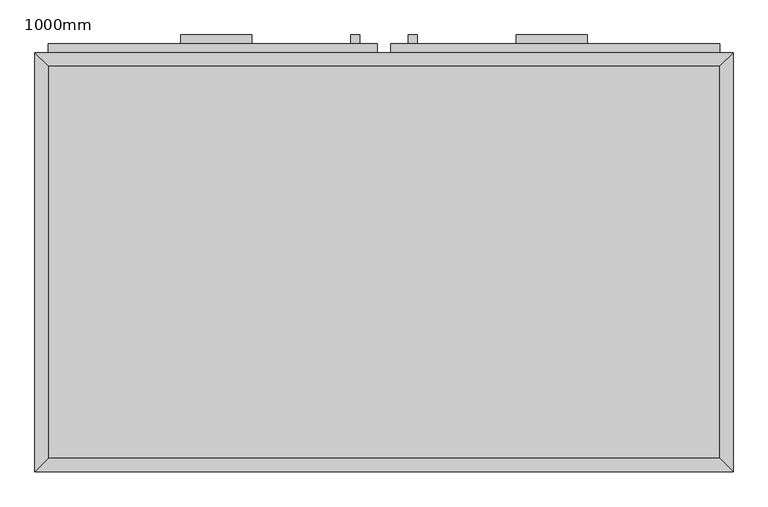
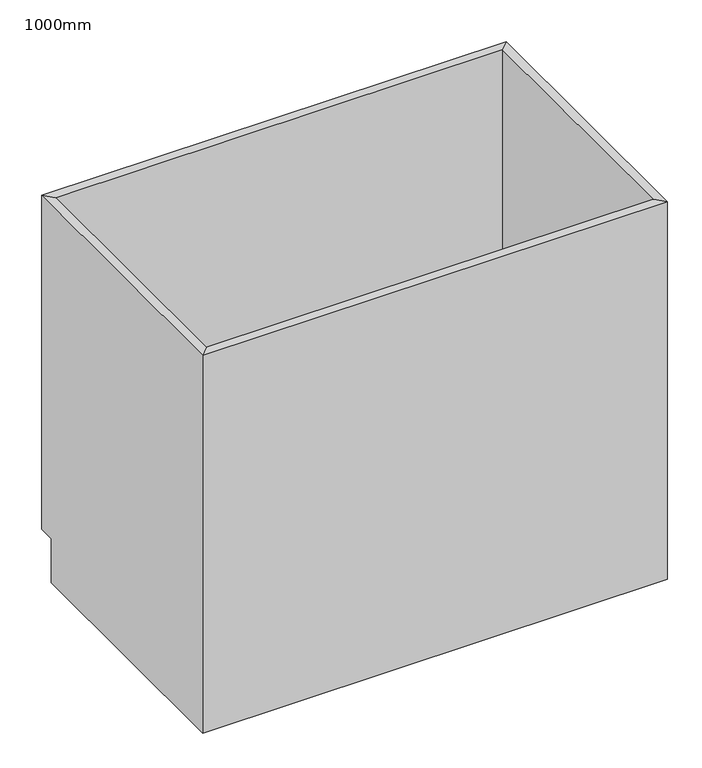
"""IFC4 building model written with IfcOpenShell, lengths in millimetres: furniture geometry, M_Base Cabinet-Double Door & 2 Drawer : 1000mm."""

from ifc_helpers import new_model, si_unit, frame, origin, place, context, project, spatial, polyline, outline, extrude, faceted_brep, source, transform, mapped, element, save


def furniture_1000mm_55825455(model_context):
    return source(origin(), model_context, "Body", "SolidModel", [
        faceted_brep([(499.6877049, 580.95, 860.0), (-462.2122951, 580.95, 860.0), (-462.2122951, 580.95, 100.0), (499.6877049, 580.95, 100.0), (518.7377049, 600.0, 860.0), (-481.2622951, 600.0, 860.0), (518.7377049, 600.0, 100.0), (-481.2622951, 600.0, 100.0), (-462.2122951, 19.05, 860.0), (-462.2122951, 19.05, 100.0), (-462.2122951, 565.0, 100.0), (-481.2622951, 0.0, 860.0), (-481.2622951, 565.0, 100.0), (-481.2622951, 565.0, 0.0), (-481.2622951, 0.0, 0.0), (499.6877049, 19.05, 860.0), (499.6877049, 19.05, 100.0), (518.7377049, 0.0, 860.0), (518.7377049, 0.0, 0.0), (499.6877049, 565.0, 100.0), (518.7377049, 565.0, 0.0), (518.7377049, 565.0, 100.0)], [[[0, 1, 2, 3]], [[0, 4, 5, 1]], [[4, 6, 7, 5]], [[2, 7, 6, 3]], [[1, 8, 9, 10, 2]], [[5, 11, 8, 1]], [[7, 12, 13, 14, 11, 5]], [[2, 10, 12, 7]], [[8, 15, 16, 9]], [[11, 17, 15, 8]], [[14, 18, 17, 11]], [[3, 19, 16, 15, 0]], [[0, 15, 17, 4]], [[4, 17, 18, 20, 21, 6]], [[6, 21, 19, 3]], [[10, 9, 16, 19]], [[18, 14, 13, 20]], [[13, 12, 10, 19, 21, 20]]]),
        extrude(outline(polyline([(-170.9372951, 625.4), (-170.9372951, 612.7), (-272.5372951, 612.7), (-272.5372951, 625.4), (-170.9372951, 625.4)])), frame((0.0, 0.0, 802.85), z_axis=(0.0, 0.0, 1.0), x_axis=(1.0, 0.0, 0.0)), (0.0, 0.0, 1.0), 12.7),
        extrude(outline(polyline([(310.0127049, 625.4), (310.0127049, 612.7), (208.4127049, 612.7), (208.4127049, 625.4), (310.0127049, 625.4)])), frame((0.0, 0.0, 802.85), z_axis=(0.0, 0.0, 1.0), x_axis=(1.0, 0.0, 0.0)), (0.0, 0.0, 1.0), 12.7),
        extrude(outline(polyline([(-16.1872951, 625.4), (-16.1872951, 612.7), (-28.8872951, 612.7), (-28.8872951, 625.4), (-16.1872951, 625.4)])), frame((0.0, 0.0, 580.6), z_axis=(0.0, 0.0, 1.0), x_axis=(1.0, 0.0, 0.0)), (0.0, 0.0, 1.0), 101.6),
        extrude(outline(polyline([(66.3627049, 625.4), (66.3627049, 612.7), (53.6627049, 612.7), (53.6627049, 625.4), (66.3627049, 625.4)])), frame((0.0, 0.0, 580.6), z_axis=(0.0, 0.0, 1.0), x_axis=(1.0, 0.0, 0.0)), (0.0, 0.0, 1.0), 101.6),
        extrude(outline(polyline([(9.2127049, 612.7), (9.2127049, 600.0), (-462.2122951, 600.0), (-462.2122951, 612.7), (9.2127049, 612.7)])), frame((0.0, 0.0, 739.35), z_axis=(0.0, 0.0, 1.0), x_axis=(1.0, 0.0, 0.0)), (0.0, 0.0, 1.0), 101.6),
        extrude(outline(polyline([(499.6877049, 612.7), (499.6877049, 600.0), (28.2627049, 600.0), (28.2627049, 612.7), (499.6877049, 612.7)])), frame((0.0, 0.0, 739.35), z_axis=(0.0, 0.0, 1.0), x_axis=(1.0, 0.0, 0.0)), (0.0, 0.0, 1.0), 101.6),
        extrude(outline(polyline([(9.2127049, 612.7), (9.2127049, 600.0), (-462.2122951, 600.0), (-462.2122951, 612.7), (9.2127049, 612.7)])), frame((0.0, 0.0, 119.05), z_axis=(0.0, 0.0, 1.0), x_axis=(1.0, 0.0, 0.0)), (0.0, 0.0, 1.0), 601.25),
        extrude(outline(polyline([(499.6877049, 612.7), (499.6877049, 600.0), (28.2627049, 600.0), (28.2627049, 612.7), (499.6877049, 612.7)])), frame((0.0, 0.0, 119.05), z_axis=(0.0, 0.0, 1.0), x_axis=(1.0, 0.0, 0.0)), (0.0, 0.0, 1.0), 601.25),
        extrude(outline(polyline([(499.6877049, 19.05), (-462.2122951, 19.05), (-462.2122951, 580.95), (499.6877049, 580.95), (499.6877049, 19.05)])), frame((0.0, 0.0, 100.0), z_axis=(0.0, 0.0, 1.0), x_axis=(1.0, 0.0, 0.0)), (0.0, 0.0, 1.0), 19.05),
    ])


if __name__ == "__main__":
    model = new_model("IFC4")
    model_context = context("Model", 3, world=origin())
    ifc_project = project(units=[si_unit("LENGTHUNIT", "METRE", prefix="MILLI")], contexts=[model_context])
    site = spatial("IfcSite", under=ifc_project)
    building = spatial("IfcBuilding", under=site)
    placement = place(None, origin())
    furniture_1000mm_shape = furniture_1000mm_55825455(model_context)
    element("IfcFurniture", 1, ObjectType="M_Base Cabinet-Double Door & 2 Drawer : 1000mm", at=placement, inside=building, context=model_context, shape_type="MappedRepresentation", body=[
        mapped(furniture_1000mm_shape, transform((0.0, 0.0, 0.0), x_axis=(1.0, 0.0, 0.0), y_axis=(0.0, 1.0, 0.0), z_axis=(0.0, 0.0, 1.0))),
    ])
    save(model, "model.ifc")

# Revit data of these elements
# Type "M_Base Cabinet-Double Door & 2 Drawer : 1000mm"
#   Manufacturer = "Manufacturer"
#   Finish = "Finish"
#   Construction Type = "Construction Type"
#   AccessibilityPerformance = "AccessibilityPerformance"
#   CodePerformance = "CodePerformance"
#   Area = "Area"
#   Color = "Color"
#   Constituents = "Constituents"
#   Features = "Features"
#   Finish = "Finish"
#   Grade = "Grade"
#   Material = "Material"
#   ModelReference = "ModelReference"
#   NominalHeight = "NominalHeight"
#   NominalLength = "NominalLength"
#   NominalWidth = "NominalWidth"
#   ProductionYear = "ProductionYear"
#   Reference = "Reference"
#   Shape = "Shape"
#   Size = "Size"
#   SustainabilityPerformance = "SustainabilityPerformance"
#   WarrantyDescription = "WarrantyDescription"
#   WarrantyDurationLabor = "WarrantyDurationLabor"
#   WarrantyDurationParts = "WarrantyDurationParts"
#   WarrantyGuarantorLabor = "WarrantyGuarantorLabor"
#   WarrantyGuarantorParts = "WarrantyGuarantorParts"
#   ExpectedLife = "ExpectedLife"
#   ReplacementCost = "ReplacementCost"
#   AssetAccountingType = "FIXED"
#   ModelLabel = "ModelLabel"
#   Depth = 0.600 m
#   Height = 0.860 m
#   Plinth Depth = 0.035 m
#   Plinth Height = 0.100 m
#   Width = 1.000 m
#   Cabinet Material = none
#   Door/Drawer Material = none
#   Handle Material = Cabinets - Handles
# Element 1 (IfcFurniture, "M_Base Cabinet-Double Door & 2 Drawer : 1000mm")
#   Materials on its faces: "Cabinets", "Cabinets - Handles"
# Materials
#   "Cabinets - Handles": class "Metal", colour RGB 57 57 57, transparency 0
#   "Cabinets": class "Miscellaneous", colour RGB 249 249 249, transparency 0
